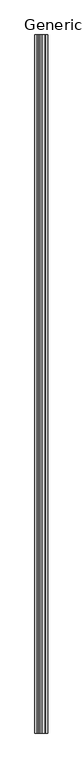
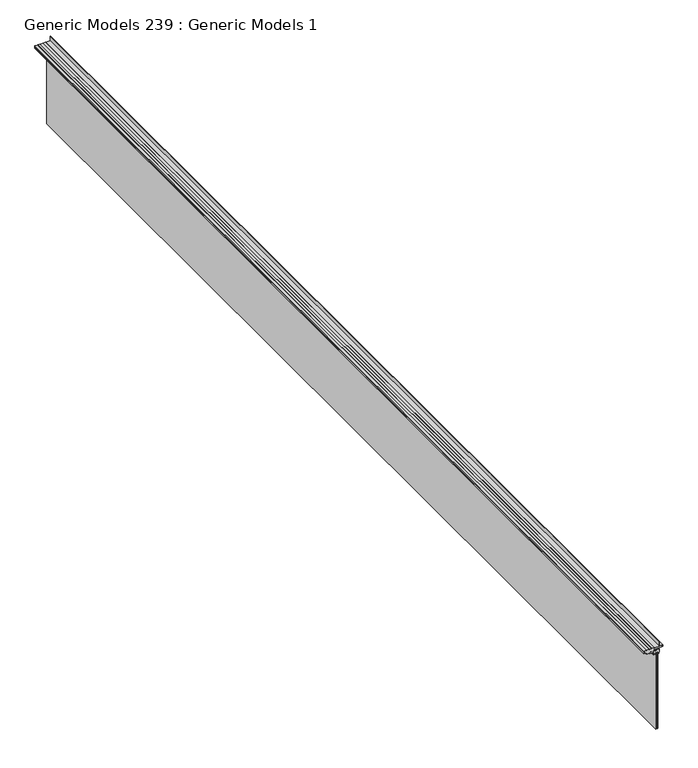
"""IFC4 building model written with IfcOpenShell, lengths in millimetres: proxy geometry, Generic Models 239 : Generic Models 1."""

from ifc_helpers import new_model, si_unit, point, frame, frame_2d, origin, place, context, project, spatial, polyline, circle_curve, trimmed, segment, composite_curve, outline, extrude, source, transform, mapped, element, save


def generic_models_239_generic_models_1_bc144803(model_context):
    return source(origin(), model_context, "Body", "SweptSolid", [
        extrude(outline(composite_curve([segment(polyline([(129382.901, 69043.6793984), (129374.9507828, 69043.6793984), (129374.9507828, 69051.6295914), (129372.9696052, 69051.6295914), (129372.9696052, 69043.6793984), (129363.0381862, 69043.6793984), (129363.0381862, 69053.9917535), (129362.2253967, 69054.7792054), (129362.2253967, 69057.9542054), (129358.2629932, 69057.9542054), (129358.2629932, 69059.5543984), (129355.0879932, 69063.4913674), (129355.0879932, 69065.0915604), (129352.7003967, 69065.0915604), (129352.7003967, 69084.1415604), (129346.3685642, 69084.1415604), (129346.3685642, 69113.5547845), (129349.5435642, 69113.5547845), (129349.5435642, 69110.5068116), (129358.2303642, 69110.5068116), (129358.2303642, 69092.9808116), (129360.5163642, 69092.9808116), (129360.5163642, 69110.5068116), (129361.4561607, 69110.5068116), (129361.4561607, 69118.9141473), (129369.4063537, 69118.9141473), (129369.4063537, 69120.8954217), (129362.9874141, 69120.8954217), (129362.9874141, 69124.9085488), (129367.8642068, 69124.9085488), (129367.8642068, 69159.8589488), (129370.2865766, 69187.7227488), (129379.218, 69187.7227488), (129379.218, 69179.8191832), (129381.504, 69179.8191832), (129381.504, 69186.1691832), (129382.901, 69186.1691832), (129382.901, 69161.2813488), (129418.268087, 69161.2813488)]), True, "CONTINUOUS"), segment(trimmed(circle_curve(frame_2d((129418.2705467, 69160.582849)), 0.6985041), [point((129418.268087, 69161.2813488))], [point((129418.2728876, 69159.8843488))], False, "CARTESIAN"), True, "CONTINUOUS"), segment(polyline([(129418.2728876, 69159.8843488), (129382.901, 69159.8843488), (129382.901, 69123.415181), (129379.726, 69123.415181), (129379.726, 69121.129181), (129382.901, 69121.129181), (129382.901, 69104.0297984), (129380.8182, 69104.0297984), (129380.8182, 69100.8547984), (129382.901, 69100.8547984), (129382.901, 69083.8276988), (129379.726, 69083.8276988), (129379.726, 69081.5416949), (129382.901, 69081.5416949), (129382.901, 69064.0339457), (129379.726, 69064.0339457), (129379.726, 69061.7479419), (129382.901, 69061.7479419), (129382.901, 69043.6793984)]), True, "CONTINUOUS")], self_intersect=False)), frame((0.0, -14323.7036701, 0.0), z_axis=(0.0, 1.0, 0.0), x_axis=(0.0, 0.0, 1.0)), (0.0, 0.0, 1.0), 7886.7),
        extrude(outline(composite_curve([segment(polyline([(129334.0440891, 69151.3824909), (129329.80865, 69151.3824909), (129329.80865, 69152.5183488), (129327.7822762, 69152.5183488), (129327.9718265, 69154.9613882), (129335.77765, 69157.4967488), (129335.77765, 69159.8843488), (129358.07885, 69159.8843488)]), True, "CONTINUOUS"), segment(trimmed(circle_curve(frame_2d((129358.07885, 69157.4967488)), 2.3876), [point((129358.07885, 69159.8843488))], [point((129360.46645, 69157.4967488))], False, "CARTESIAN"), True, "CONTINUOUS"), segment(polyline([(129360.46645, 69157.4967488), (129360.46645, 69154.9313488), (129358.43445, 69154.9313488), (129358.43445, 69153.2549488), (129355.13245, 69153.2549488), (129355.13245, 69151.3499488), (129363.05725, 69151.3499488), (129363.05725, 69145.7365488), (129357.74865, 69145.7365488), (129357.74865, 69133.5445488)]), True, "CONTINUOUS"), segment(trimmed(circle_curve(frame_2d((129357.74865, 69131.5633488)), 1.9812), [point((129357.74865, 69133.5445488))], [point((129357.74865, 69129.5821488))], True, "CARTESIAN"), True, "CONTINUOUS"), segment(polyline([(129357.74865, 69129.5821488), (129357.74865, 69116.2471488)]), True, "CONTINUOUS"), segment(trimmed(circle_curve(frame_2d((129356.93585, 69116.2471488)), 0.8128), [point((129357.74865, 69116.2471488))], [point((129356.93585, 69115.4343488))], False, "CARTESIAN"), True, "CONTINUOUS"), segment(polyline([(129356.93585, 69115.4343488), (129338.64785, 69115.4343488), (129338.64785, 69117.3148668), (129337.0469612, 69117.3148668), (129337.0469612, 69115.7146668), (129329.5031612, 69115.7146668), (129329.5031612, 69119.4825863), (129327.3408112, 69119.4825863), (129326.3281612, 69131.3102668), (129336.2595612, 69131.3102668), (129338.64785, 69128.921978), (129338.64785, 69150.3593488), (129335.0672312, 69150.3593488), (129334.0440891, 69151.3824909)]), True, "CONTINUOUS")], self_intersect=False)), frame((0.0, -14323.7036701, 0.0), z_axis=(0.0, 1.0, 0.0), x_axis=(0.0, 0.0, 1.0)), (0.0, 0.0, 1.0), 7886.7),
        extrude(outline(polyline([(69136.8665168, -14323.7036701), (69132.1040168, -14323.7036701), (69132.1040168, -6437.0036701), (69136.8665168, -6437.0036701), (69136.8665168, -14323.7036701)])), frame((0.0, 0.0, 128735.5165519), z_axis=(0.0, 0.0, 1.0), x_axis=(1.0, 0.0, 0.0)), (0.0, 0.0, 1.0), 602.3375481),
        extrude(outline(polyline([(69144.0093488, -14323.7036701), (69137.6602668, -14323.7036701), (69137.6602668, -6437.0036701), (69144.0093488, -6437.0036701), (69144.0093488, -14323.7036701)])), frame((0.0, 0.0, 129331.5041), z_axis=(0.0, 0.0, 1.0), x_axis=(1.0, 0.0, 0.0)), (0.0, 0.0, 1.0), 6.35),
        extrude(outline(polyline([(69149.5655988, -14323.7036701), (69144.8030988, -14323.7036701), (69144.8030988, -6437.0036701), (69149.5655988, -6437.0036701), (69149.5655988, -14323.7036701)])), frame((0.0, 0.0, 128735.5165519), z_axis=(0.0, 0.0, 1.0), x_axis=(1.0, 0.0, 0.0)), (0.0, 0.0, 1.0), 602.3375481),
    ])


if __name__ == "__main__":
    model = new_model("IFC4")
    model_context = context("Model", 3, world=origin())
    ifc_project = project(units=[si_unit("LENGTHUNIT", "METRE", prefix="MILLI")], contexts=[model_context])
    site = spatial("IfcSite", under=ifc_project)
    building = spatial("IfcBuilding", under=site)
    placement = place(None, origin())
    generic_models_239_generic_models_1_shape = generic_models_239_generic_models_1_bc144803(model_context)
    element("IfcBuildingElementProxy", 1, Name="Generic Models 239 : Generic Models 1", ObjectType="Generic Models 239 : Generic Models 1", at=placement, inside=building, context=model_context, shape_type="MappedRepresentation", body=[
        mapped(generic_models_239_generic_models_1_shape, transform((0.0, 0.0, 0.0), x_axis=(1.0, 0.0, 0.0), y_axis=(0.0, 1.0, 0.0), z_axis=(0.0, 0.0, 1.0))),
    ])
    save(model, "model.ifc")

# Revit data of these elements
# Element 1 (IfcBuildingElementProxy, "Generic Models 239 : Generic Models 1")
#   Materials on its faces: "_WINDOW PER SCHEDULE"
# Materials
#   "_WINDOW PER SCHEDULE": class "Generic", colour RGB 255 255 255, transparency 0, Cost = 0
